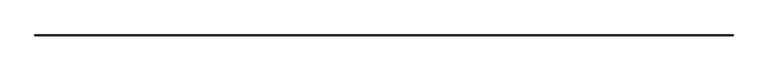
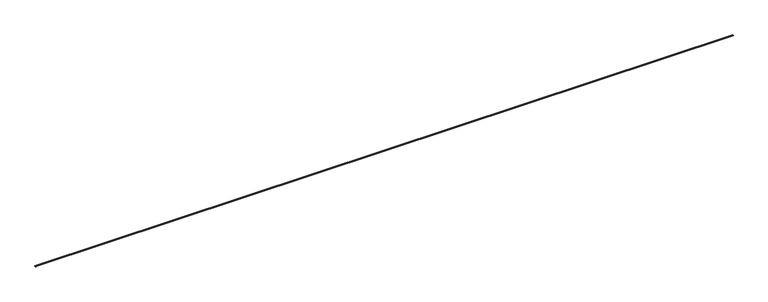
"""IFC4 building model written with IfcOpenShell, lengths in millimetres: proxy geometry, Generic Models 3:Generic Models 1:4:Generic Models 1:4 : Generic Models 3:Generic Models 1:300625:1:Generic Models 1:4:Generic Models 1:4 : Generic Models 3:Generic Models 1:300625:1 : Generic Models 3:Generic Models 1:4:Generic Models 1:4 : Generic Models 3:Generic Models 1:300625:338780:2 : Generic Models 3:Generic Models 1:4:Generic Models 1:4 : Generic Models 3:Generic Models 1:300625:1:Generic Models 1:4:Generic Models 1:4 : Generic Models 3:Generic Models 1:300625:1 : Generic Models 3:Generic Models 1:4:Generic Models 1:4 : Generic Models 3:Generic Models 1:300625:338780:317135."""

from ifc_helpers import new_model, si_unit, frame, origin, place, context, project, spatial, polyline, outline, extrude, source, transform, mapped, element, save


def generic_models_aa0125ff(model_context):
    return source(origin(), model_context, "Body", "SweptSolid", [
        extrude(outline(polyline([(-579088.4739295, 3713.8232545), (-579094.6612723, 3713.8232545), (-579094.1146795, 3714.4746585), (-579093.8638533, 3715.4107545), (-579094.1146795, 3716.3468505), (-579094.6612723, 3716.9982545), (-579088.4739295, 3716.9982545), (-579089.0205223, 3716.3468505), (-579089.2713485, 3715.4107545), (-579089.0205223, 3714.4746585), (-579088.4739295, 3713.8232545)])), frame((591306.0367239, 0.0, 0.0), z_axis=(1.0, 0.0, 0.0), x_axis=(0.0, 1.0, 0.0)), (0.0, 0.0, 1.0), 4876.8),
    ])


if __name__ == "__main__":
    model = new_model("IFC4")
    model_context = context("Model", 3, world=origin())
    ifc_project = project(units=[si_unit("LENGTHUNIT", "METRE", prefix="MILLI")], contexts=[model_context])
    site = spatial("IfcSite", under=ifc_project)
    building = spatial("IfcBuilding", under=site)
    placement = place(None, origin())
    generic_models_shape = generic_models_aa0125ff(model_context)
    element("IfcBuildingElementProxy", 1, Name="Generic Models 3:Generic Models 1:4:Generic Models 1:4 : Generic Models 3:Generic Models 1:300625:1:Generic Models 1:4:Generic Models 1:4 : Generic Models 3:Generic Models 1:300625:1 : Generic Models 3:Generic Models 1:4:Generic Models 1:4 : Generic Models 3:Generic Models 1:300625:338780:2 : Generic Models 3:Generic Models 1:4:Generic Models 1:4 : Generic Models 3:Generic Models 1:300625:1:Generic Models 1:4:Generic Models 1:4 : Generic Models 3:Generic Models 1:300625:1 : Generic Models 3:Generic Models 1:4:Generic Models 1:4 : Generic Models 3:Generic Models 1:300625:338780:317135", ObjectType="Generic Models 3:Generic Models 1:4:Generic Models 1:4 : Generic Models 3:Generic Models 1:300625:1:Generic Models 1:4:Generic Models 1:4 : Generic Models 3:Generic Models 1:300625:1 : Generic Models 3:Generic Models 1:4:Generic Models 1:4 : Generic Models 3:Generic Models 1:300625:338780:2 : Generic Models 3:Generic Models 1:4:Generic Models 1:4 : Generic Models 3:Generic Models 1:300625:1:Generic Models 1:4:Generic Models 1:4 : Generic Models 3:Generic Models 1:300625:1 : Generic Models 3:Generic Models 1:4:Generic Models 1:4 : Generic Models 3:Generic Models 1:300625:338780:317135", at=placement, inside=building, context=model_context, shape_type="MappedRepresentation", body=[
        mapped(generic_models_shape, transform((0.0, 0.0, 0.0), x_axis=(1.0, 0.0, 0.0), y_axis=(0.0, 1.0, 0.0), z_axis=(0.0, 0.0, 1.0))),
    ])
    save(model, "model.ifc")

# Revit data of these elements
# Type "Generic Models 3:Generic Models 1:4:Generic Models 1:4 : Generic Models 3:Generic Models 1:300625:1:Generic Models 1:4:Generic Models 1:4 : Generic Models 3:Generic Models 1:300625:1 : Generic Models 3:Generic Models 1:4:Generic Models 1:4 : Generic Models 3:Generic Models 1:300625:338780:2 : Generic Models 3:Generic Models 1:4:Generic Models 1:4 : Generic Models 3:Generic Models 1:300625:1:Generic Models 1:4:Generic Models 1:4 : Generic Models 3:Generic Models 1:300625:1 : Generic Models 3:Generic Models 1:4:Generic Models 1:4 : Generic Models 3:Generic Models 1:300625:338780:317135"
#   NameOverride = "Generic Models 3:Generic Models 1:4:Generic Models 1:4 : Generic Models 3:Generic Models 1:300625:1:Generic Models 1:4:Generic Models 1:4 : Generic Models 3:Generic Models 1:300625:1 : Generic Models 3:Generic Models 1:4:Generic Models 1:4 : Generic Models 3:Generic Models 1:300625:338780:317135"
#   ObjectTypeOverride = "Generic Models 1:4:Generic Models 1:4 : Generic Models 3:Generic Models 1:300625:1 : Generic Models 3:Generic Models 1:4:Generic Models 1:4 : Generic Models 3:Generic Models 1:300625:338780"
#   Reference = "Generic Models 1"
#   Tag = "317135"
# Element 1 (IfcBuildingElementProxy, "Generic Models 3:Generic Models 1:4:Generic Models 1:4 : Generic Models 3:Generic Models 1:300625:1:Generic Models 1:4:Generic Models 1:4 : Generic Models 3:Generic Models 1:300625:1 : Generic Models 3:Generic Models 1:4:Generic Models 1:4 : Generic Models 3:Generic Models 1:300625:338780:2 : Generic Models 3:Generic Models 1:4:Generic Models 1:4 : Generic Models 3:Generic Models 1:300625:1:Generic Models 1:4:Generic Models 1:4 : Generic Models 3:Generic Models 1:300625:1 : Generic Models 3:Generic Models 1:4:Generic Models 1:4 : Generic Models 3:Generic Models 1:300625:338780:317135")
#   Materials on its faces: "SEALANT & BACKER ROD, IF NECESSARY"
# Materials
#   "SEALANT & BACKER ROD, IF NECESSARY": class "Unassigned", colour RGB 120 120 120, transparency 0, Cost = 0
